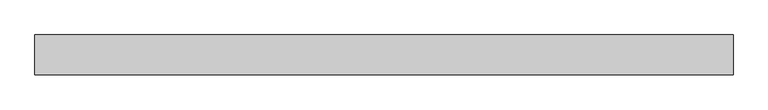
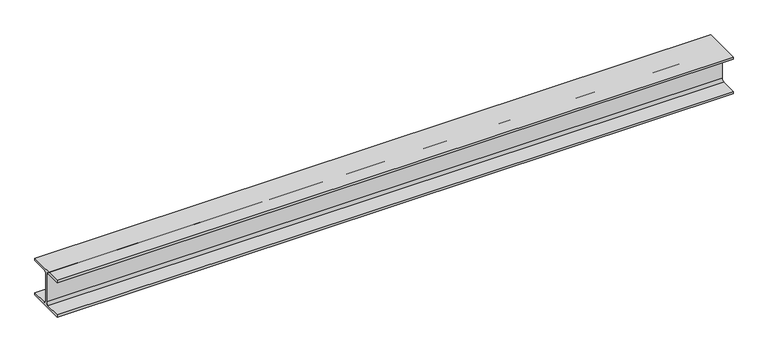
"""IFC4 building model written with IfcOpenShell, lengths in millimetres: beam geometry, 0912_Steel Framing_H-KSD3502 : H_SB_ASB_H-200x200x8x12."""

from ifc_helpers import new_model, si_unit, point, frame, frame_2d, origin, place, context, project, spatial, polyline, circle_curve, trimmed, segment, composite_curve, outline, extrude, source, transform, mapped, element, save


def beam_35326c69(model_context):
    return source(origin(), model_context, "Body", "SweptSolid", [
        extrude(outline(composite_curve([segment(polyline([(-100.0, -88.0), (-17.0, -88.0)]), True, "CONTINUOUS"), segment(trimmed(circle_curve(frame_2d((-17.0, -75.0)), 13.0), [point((-17.0, -88.0))], [point((-4.0, -75.0))], True, "CARTESIAN"), True, "CONTINUOUS"), segment(polyline([(-4.0, -75.0), (-4.0, 75.0)]), True, "CONTINUOUS"), segment(trimmed(circle_curve(frame_2d((-17.0, 75.0)), 13.0), [point((-4.0, 75.0))], [point((-17.0, 88.0))], True, "CARTESIAN"), True, "CONTINUOUS"), segment(polyline([(-17.0, 88.0), (-100.0, 88.0), (-100.0, 100.0), (100.0, 100.0), (100.0, 88.0), (17.0, 88.0)]), True, "CONTINUOUS"), segment(trimmed(circle_curve(frame_2d((17.0, 75.0)), 13.0), [point((17.0, 88.0))], [point((4.0, 75.0))], True, "CARTESIAN"), True, "CONTINUOUS"), segment(polyline([(4.0, 75.0), (4.0, -75.0)]), True, "CONTINUOUS"), segment(trimmed(circle_curve(frame_2d((17.0, -75.0)), 13.0), [point((4.0, -75.0))], [point((17.0, -88.0))], True, "CARTESIAN"), True, "CONTINUOUS"), segment(polyline([(17.0, -88.0), (100.0, -88.0), (100.0, -100.0), (-100.0, -100.0), (-100.0, -88.0)]), True, "CONTINUOUS")], self_intersect=False)), frame((-1763.3300108, 0.0, 0.0), z_axis=(1.0, 0.0, 0.0), x_axis=(0.0, 1.0, 0.0)), (0.0, 0.0, 1.0), 3493.2799911),
    ])


if __name__ == "__main__":
    model = new_model("IFC4")
    model_context = context("Model", 3, world=origin())
    ifc_project = project(units=[si_unit("LENGTHUNIT", "METRE", prefix="MILLI")], contexts=[model_context])
    site = spatial("IfcSite", under=ifc_project)
    building = spatial("IfcBuilding", under=site)
    placement = place(None, origin())
    beam_shape = beam_35326c69(model_context)
    element("IfcBeam", 1, ObjectType="0912_Steel Framing_H-KSD3502 : H_SB_ASB_H-200x200x8x12", at=placement, inside=building, context=model_context, shape_type="MappedRepresentation", body=[
        mapped(beam_shape, transform((0.0, 0.0, 0.0), x_axis=(1.0, 0.0, 0.0), y_axis=(0.0, 1.0, 0.0), z_axis=(0.0, 0.0, 1.0))),
    ])
    save(model, "model.ifc")

# Revit data of these elements
# Type "0912_Steel Framing_H-KSD3502 : H_SB_ASB_H-200x200x8x12"
#   H_WM Code_1 = "S01AA002-00001 | Main Steel Structure Fabrication Work | Shelter/Building | Medium Steel - Standard (90KG/M>Weight≥30KG/M) | Material: (   )"
#   H_WM Code_2 = "S03AA028-00001 | Main Steel Structure Erection Work | Shelter/Building | Medium Steel (90KG/M>Weight≥30KG/M) | Material: (   )"
#   H_WM Code_3 = "S01AA010-00001 | Main Steel Structure Fabrication Work | Shelter/Building | Steel Painting/Coating | for Non-Fireproofed Steel Surface, Surface Preparation, Primer, Second & Final Coat | Material: (   )"
#   H_Q'ty Cal Type Tag = "SB-Q2"
#   Width = 20.0 cm
#   Web Thickness = 0.8 cm
#   Web Fillet = 1.3 cm
#   Warping Constant = 141000.0 cm⁶
#   W = 0
#   Torsional Moment of Inertia = 26.2485 cm⁴
#   Section Area = 63.53 cm²
#   Plastic Modulus weak axis = 244.0 cm³
#   Plastic Modulus strong axis = 525.0 cm³
#   Perimeter = 1.16 m²/m
#   Nominal Weight = 49.90 kgf/m
#   Moment of Inertia weak axis = 1600.00 cm⁴
#   Moment of Inertia strong axis = 4720.00 cm⁴
#   Height = 20.0 cm
#   Flange Thickness = 1.2 cm
#   Elastic Modulus weak axis = 160.0 cm³
#   Elastic Modulus strong axis = 472.0 cm³
#   Centroid Vertical = 10.0 cm
#   Centroid Horizontal = 10.0 cm
#   Ix = 47200000
#   Length [instance default] = 1.5240 m
#   Zx = 525000
#   b = 0.2000 m
#   h = 0.2000 m
#   r = 0.0130 m
#   s = 0.0080 m
#   t = 0.0120 m
#   A = 0.006353 m²
#   Structural Material [instance default] = Steel, 45-345
#   Assembly Code = ""
# Element 1 (IfcBeam, "0912_Steel Framing_H-KSD3502 : H_SB_ASB_H-200x200x8x12")
#   Structural Material = none
# Materials
#   "Steel, 45-345": class "Metal", colour RGB 189 187 185, transparency 0, Description = "Steel 345 MPa", Cost = 0
